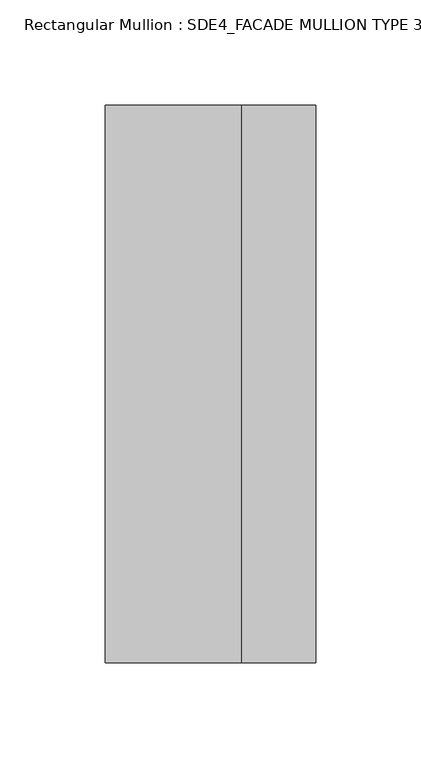
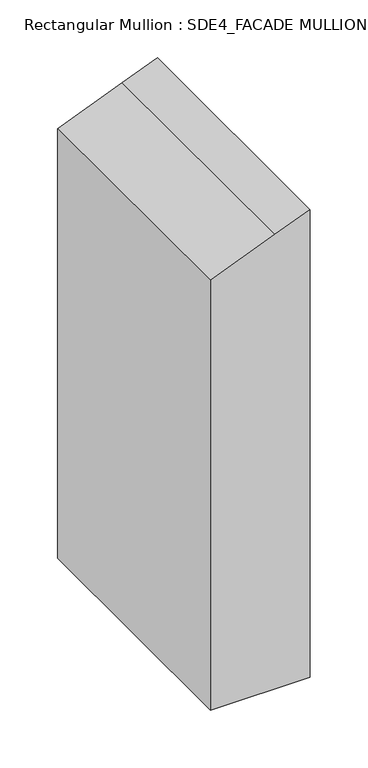
"""IFC4 building model written with IfcOpenShell, lengths in millimetres: member geometry, Rectangular Mullion : SDE4_FACADE MULLION TYPE 3."""

from ifc_helpers import new_model, si_unit, frame, origin, place, context, project, spatial, polyline, outline, extrude, source, transform, mapped, element, save


def rectangular_mullion_sde4_facade_mullion_type_3_7fc80fe7(model_context):
    return source(origin(), model_context, "Body", "SweptSolid", [
        extrude(outline(polyline([(-23.0813185, 50.0), (-37.1390676, 14.8556271), (-63.0813185, -50.0), (-517.974544, -50.0), (-517.974544, 50.0), (-23.0813185, 50.0)])), frame((0.0, -132.5, 0.0), z_axis=(0.0, 1.0, 0.0), x_axis=(0.0, 0.0, 1.0)), (0.0, 0.0, 1.0), 265.0),
    ])


if __name__ == "__main__":
    model = new_model("IFC4")
    model_context = context("Model", 3, world=origin())
    ifc_project = project(units=[si_unit("LENGTHUNIT", "METRE", prefix="MILLI")], contexts=[model_context])
    site = spatial("IfcSite", under=ifc_project)
    building = spatial("IfcBuilding", under=site)
    placement = place(None, origin())
    rectangular_mullion_sde4_facade_mullion_type_3_shape = rectangular_mullion_sde4_facade_mullion_type_3_7fc80fe7(model_context)
    element("IfcMember", 1, ObjectType="Rectangular Mullion : SDE4_FACADE MULLION TYPE 3", at=placement, inside=building, context=model_context, shape_type="MappedRepresentation", body=[
        mapped(rectangular_mullion_sde4_facade_mullion_type_3_shape, transform((0.0, 0.0, 0.0), x_axis=(1.0, 0.0, 0.0), y_axis=(0.0, 1.0, 0.0), z_axis=(0.0, 0.0, 1.0))),
    ])
    save(model, "model.ifc")

# Revit data of these elements
# Type "Rectangular Mullion : SDE4_FACADE MULLION TYPE 3"
#   built-in parameter 1007322 = 0.869423 (stored number, unit not read)
#   built-in parameter 1007321 = 0.164042 (stored number, unit not read)
#   built-in parameter 1007320 = 0.164042 (stored number, unit not read)
